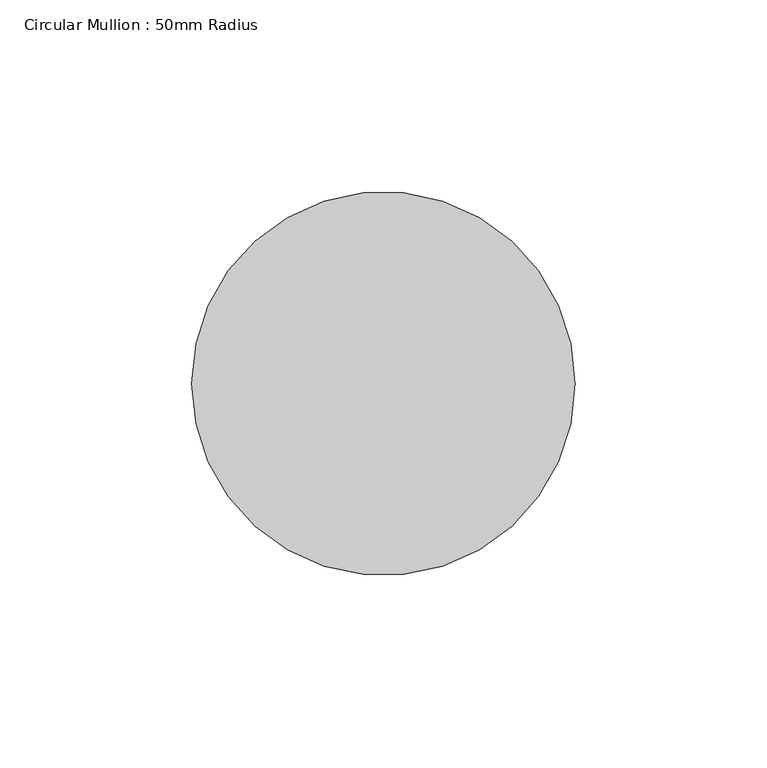
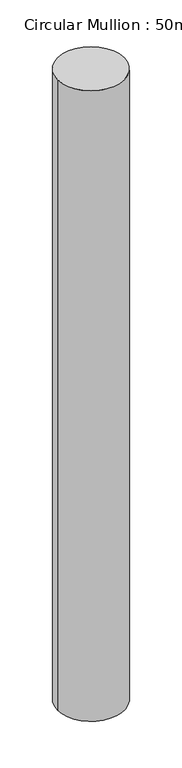
"""IFC4 building model written with IfcOpenShell, lengths in millimetres: member geometry, Circular Mullion : 50mm Radius."""

from ifc_helpers import new_model, si_unit, point, frame, origin, origin_2d, place, context, project, spatial, circle_curve, trimmed, segment, composite_curve, outline, extrude, source, transform, mapped, element, save


def circular_mullion_50mm_radius_b1944cf1(model_context):
    return source(origin(), model_context, "Body", "SweptSolid", [
        extrude(outline(composite_curve([segment(trimmed(circle_curve(origin_2d(), 50.0), [point((50.0, 0.0))], [point((-50.0, 0.0))], False, "CARTESIAN"), True, "CONTINUOUS"), segment(trimmed(circle_curve(origin_2d(), 50.0), [point((-50.0, 0.0))], [point((50.0, 0.0))], False, "CARTESIAN"), True, "CONTINUOUS")], self_intersect=False)), frame((0.0, 0.0, -998.8786604), z_axis=(0.0, 0.0, 1.0), x_axis=(1.0, 0.0, 0.0)), (0.0, 0.0, 1.0), 998.8786604),
    ])


if __name__ == "__main__":
    model = new_model("IFC4")
    model_context = context("Model", 3, world=origin())
    ifc_project = project(units=[si_unit("LENGTHUNIT", "METRE", prefix="MILLI")], contexts=[model_context])
    site = spatial("IfcSite", under=ifc_project)
    building = spatial("IfcBuilding", under=site)
    placement = place(None, origin())
    circular_mullion_50mm_radius_shape = circular_mullion_50mm_radius_b1944cf1(model_context)
    element("IfcMember", 1, ObjectType="Circular Mullion : 50mm Radius", at=placement, inside=building, context=model_context, shape_type="MappedRepresentation", body=[
        mapped(circular_mullion_50mm_radius_shape, transform((0.0, 0.0, 0.0), x_axis=(1.0, 0.0, 0.0), y_axis=(0.0, 1.0, 0.0), z_axis=(0.0, 0.0, 1.0))),
    ])
    save(model, "model.ifc")

# Revit data of these elements
# Type "Circular Mullion : 50mm Radius"
#   built-in parameter 1007350 = 0.164042 (stored number, unit not read)
# Element 1 (IfcMember, "Circular Mullion : 50mm Radius")
#   Materials on its faces: "Aluminium"
# Materials
#   "Aluminium": class "Metal", colour RGB 247 247 247, transparency 0, Description = "Aluminium 6061", Cost = 0
